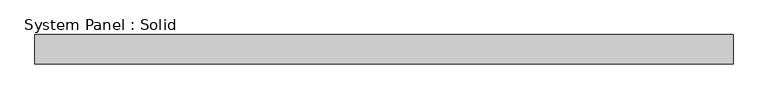
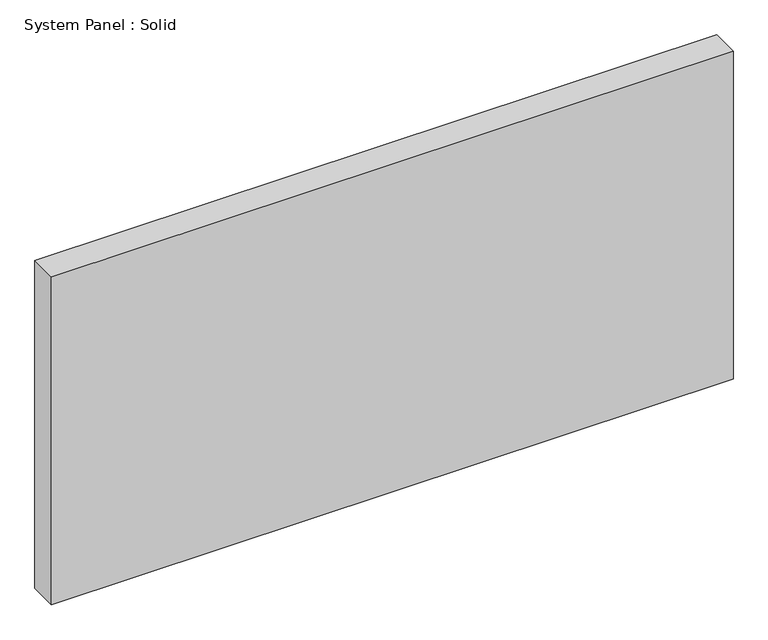
"""IFC4 building model written with IfcOpenShell, lengths in millimetres: plate geometry, System Panel : Solid."""

from ifc_helpers import new_model, si_unit, origin, origin_with_axes, place, context, project, spatial, polyline, outline, extrude, source, transform, mapped, element, save


def system_panel_solid_53db45a5(model_context):
    return source(origin(), model_context, "Body", "SweptSolid", [
        extrude(outline(polyline([(712.5, -49.5), (-712.5, -49.5), (-712.5, 10.5), (712.5, 10.5), (712.5, -49.5)])), origin_with_axes(), (0.0, 0.0, 1.0), 725.0),
    ])


if __name__ == "__main__":
    model = new_model("IFC4")
    model_context = context("Model", 3, world=origin())
    ifc_project = project(units=[si_unit("LENGTHUNIT", "METRE", prefix="MILLI")], contexts=[model_context])
    site = spatial("IfcSite", under=ifc_project)
    building = spatial("IfcBuilding", under=site)
    placement = place(None, origin())
    system_panel_solid_shape = system_panel_solid_53db45a5(model_context)
    element("IfcPlate", 1, ObjectType="System Panel : Solid", at=placement, inside=building, context=model_context, shape_type="MappedRepresentation", body=[
        mapped(system_panel_solid_shape, transform((0.0, 0.0, 0.0), x_axis=(1.0, 0.0, 0.0), y_axis=(0.0, 1.0, 0.0), z_axis=(0.0, 0.0, 1.0))),
    ])
    save(model, "model.ifc")

# Revit data of these elements
# Type "System Panel : Solid"
#   Keynote = "H11"
#   Construction Type Id = "MDOOR"
#   Analytic Construction = "Metal"
#   Visual Light Transmittance = 0
#   Solar Heat Gain Coefficient = 0
#   Heat Transfer Coefficient (U) = 3.7021 W/(m²·K)
# Element 1 (IfcPlate, "System Panel : Solid")
#   Materials on its faces: "Default"
# Materials
#   "Default": class "Miscellaneous", colour RGB 127 127 127, transparency 0, Comments = "Rendering appearance not upgraded ", Cost = 0
